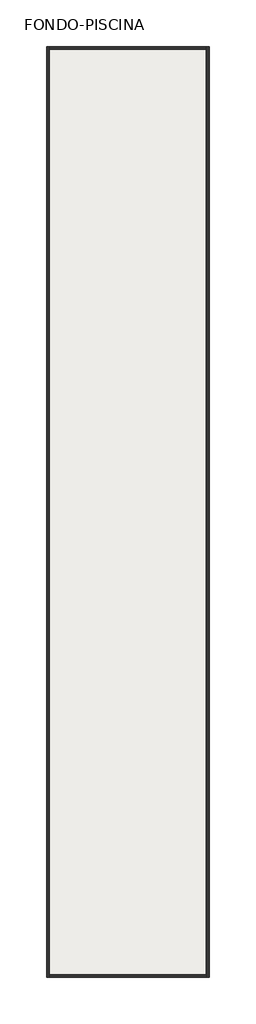
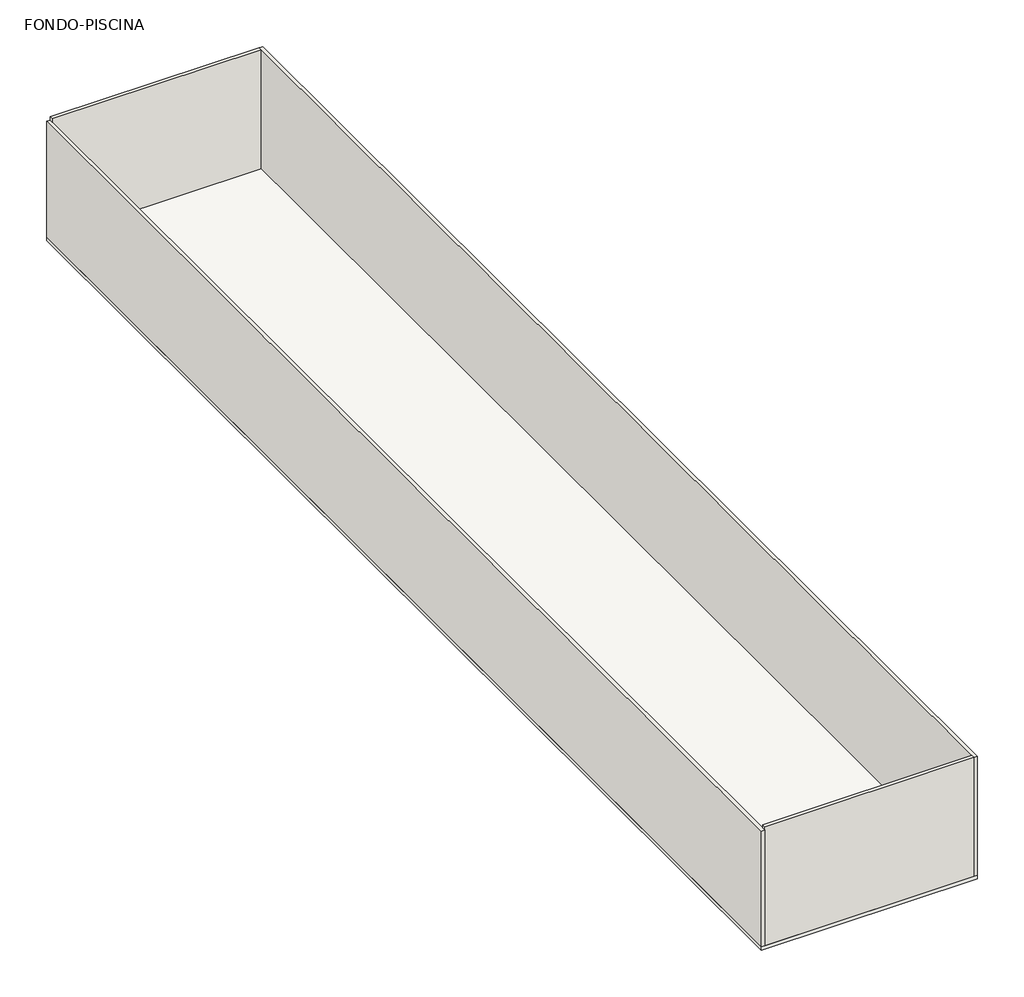
# One storey: 4 walls, 1 slab.
"""IFC4 building model written with IfcOpenShell, lengths in millimetres."""

from ifc_helpers import new_model, si_unit, origin, place, context, project, spatial, faceted_brep, element, save

model = new_model("IFC4")

# Units and contexts
model_context = context("Model", 3, world=origin())
ifc_project = project(units=[si_unit("LENGTHUNIT", "METRE", prefix="MILLI")], contexts=[model_context])

# Site, building, storey
site = spatial("IfcSite", under=ifc_project)
building = spatial("IfcBuilding", under=site)
storey = spatial("IfcBuildingStorey", under=building, Name="FONDO-PISCINA", Elevation=-1800.0)

# Slab
placement = place(None, origin())
element("IfcSlab", 1, ObjectType="ACABADO SUELO VASO PISC_PABLO", at=placement, inside=storey, context=model_context, shape_type="Brep", body=[
    faceted_brep([(-32840.0, -152.5, -1850.0), (-29750.0, -152.5, -1850.0), (-29750.0, -17847.5, -1850.0), (-32840.0, -17847.5, -1850.0), (-32840.0, -152.5, -1800.0), (-32840.0, -17847.5, -1800.0), (-32790.0, -17847.5, -1800.0), (-29800.0, -17847.5, -1800.0), (-29750.0, -17847.5, -1800.0), (-29750.0, -152.5, -1800.0), (-29800.0, -152.5, -1800.0), (-32790.0, -152.5, -1800.0)], [[[0, 1, 2, 3]], [[4, 5, 6, 7, 8, 9, 10, 11]], [[1, 0, 4, 11, 10, 9]], [[3, 2, 8, 7, 6, 5]], [[2, 1, 9, 8]], [[0, 3, 5, 4]]]),
])

# Walls
element("IfcWall", 2, ObjectType="ACABADO MURO VASO PISCINA_PABLO", at=placement, inside=storey, context=model_context, shape_type="Brep", body=[
    faceted_brep([(-29750.0, -17847.5, -1800.0), (-29750.0, -152.5, -1800.0), (-29750.0, -152.5, 0.0), (-29750.0, -17847.5, 0.0), (-29800.0, -17847.5, -1800.0), (-29800.0, -17847.5, 0.0), (-29800.0, -17797.5, 0.0), (-29800.0, -202.5, 0.0), (-29800.0, -152.5, 0.0), (-29800.0, -152.5, -1800.0), (-29800.0, -202.5, -1800.0), (-29800.0, -17797.5, -1800.0)], [[[0, 1, 2, 3]], [[4, 5, 6, 7, 8, 9, 10, 11]], [[1, 0, 4, 11, 10, 9]], [[2, 1, 9, 8]], [[3, 2, 8, 7, 6, 5]], [[0, 3, 5, 4]]]),
])
element("IfcWall", 3, ObjectType="ACABADO MURO VASO PISCINA_PABLO", at=placement, inside=storey, context=model_context, shape_type="Brep", body=[
    faceted_brep([(-29800.0, -17847.5, 0.0), (-32790.0, -17847.5, 0.0), (-32790.0, -17847.5, -50.0), (-32790.0, -17847.5, -1800.0), (-29800.0, -17847.5, -1800.0), (-32790.0, -17797.5, 0.0), (-29800.0, -17797.5, 0.0), (-29800.0, -17797.5, -1800.0), (-32790.0, -17797.5, -1800.0)], [[[0, 1, 2, 3, 4]], [[5, 6, 7, 8]], [[1, 0, 6, 5]], [[4, 3, 8, 7]], [[6, 0, 4, 7]], [[1, 5, 8, 3, 2]]]),
])
element("IfcWall", 4, ObjectType="ACABADO MURO VASO PISCINA_PABLO", at=placement, inside=storey, context=model_context, shape_type="Brep", body=[
    faceted_brep([(-29800.0, -202.5, 0.0), (-32790.0, -202.5, 0.0), (-32790.0, -202.5, -1800.0), (-29800.0, -202.5, -1800.0), (-32790.0, -152.5, 0.0), (-29800.0, -152.5, 0.0), (-29800.0, -152.5, -1800.0), (-32790.0, -152.5, -1800.0), (-32790.0, -152.5, -50.0)], [[[0, 1, 2, 3]], [[4, 5, 6, 7, 8]], [[1, 0, 5, 4]], [[3, 2, 7, 6]], [[5, 0, 3, 6]], [[1, 4, 8, 7, 2]]]),
])
element("IfcWall", 5, ObjectType="ACABADO MURO VASO PISCINA_PABLO", at=placement, inside=storey, context=model_context, shape_type="Brep", body=[
    faceted_brep([(-32790.0, -17847.5, -1800.0), (-32790.0, -17797.5, -1800.0), (-32790.0, -202.5, -1800.0), (-32790.0, -152.5, -1800.0), (-32790.0, -152.5, -50.0), (-32790.0, -17847.5, -50.0), (-32840.0, -17847.5, -1800.0), (-32840.0, -17847.5, -50.0), (-32840.0, -152.5, -50.0), (-32840.0, -152.5, -1800.0)], [[[0, 1, 2, 3, 4, 5]], [[6, 7, 8, 9]], [[3, 2, 1, 0, 6, 9]], [[4, 3, 9, 8]], [[5, 4, 8, 7]], [[0, 5, 7, 6]]]),
])

save(model, "model.ifc")

# Revit data of these elements
# Project information
#   Fecha de emisión de proyecto = "Fecha de emisión"
#   Estado de proyecto = "Estado de proyecto"
#   Nombre de cliente = "Propietario"
#   Dirección de proyecto = "Introduzca dirección aquí"
#   Nombre de proyecto = "Nombre de proyecto"
#   Número de proyecto = "0001"
# Grids (mm)
#   "10": line (-29500, 9189.325) -> (-29500, -29213.653)
#   "1": line (-33000, 9189.325) -> (-33000, -29213.653)
#   "B": line (7688.401, -13500) -> (-37134.551, -13500)
#   "A": line (7688.401, -18000) -> (-37134.551, -18000)
#   "BC": line (7688.401, -9000) -> (-37134.551, -9000)
#   "C": line (7688.401, -4500) -> (-37134.551, -4500)
#   "D": line (7688.401, 0) -> (-37134.551, 0)
#   "6": line (0, 9189.325) -> (0, -29213.653)
#   "56": line (-6000, 9189.325) -> (-6000, -29213.653)
#   "5": line (-9000, 9189.325) -> (-9000, -29213.653)
#   "4": line (-12000, 9189.325) -> (-12000, -29213.653)
#   "3": line (-21000, 9189.325) -> (-21000, -29213.653)
#   "2": line (-24000, 9189.325) -> (-24000, -29213.653)
#   "12": line (-27000, 9189.325) -> (-27000, -29213.653)
# Type "ACABADO SUELO VASO PISC_PABLO"
#   Keynote = "S.4.2"
#   Function = 0
#   Layers, outside or top first: 0.03 m "Piedra caliza acabado" (function 5); 0.02 m "Mortero agarre" (function 4)
# Type "ACABADO MURO VASO PISCINA_PABLO"
#   Keynote = "Me.1.1"
#   Layers, outside or top first: 0.03 m "Piedra caliza acabado" (function 5); 0.02 m "Mortero agarre" (function 4); 0.00 m "Membrana impermeabilizante" (function 100)
# Element 1 (IfcSlab, "ACABADO SUELO VASO PISC_PABLO")
#   Comments = ""
#   built-in parameter 1001955 = 3.14159 (stored number, unit not read)
#   Height Offset From Level = 0.00 m
#   built-in parameter 1001954 = 1
#   Phase Created = Nueva construcción
#   Materials on its faces: "Mortero agarre", "Piedra caliza acabado"
# Element 2 (IfcWall, "ACABADO MURO VASO PISCINA_PABLO")
#   Top Offset = 0.00 m
#   Base Offset = 0.00 m
#   wall height = 1.80 m
#   Phase Created = Nueva construcción
#   Base Constraint = FONDO-PISCINA
#   Top Constraint = ACCESO
#   Materials on its faces: "Piedra caliza acabado", "Mortero agarre"
# Elements 3, 4 (IfcWall, "ACABADO MURO VASO PISCINA_PABLO")
#   built-in parameter 1001111 = -0.05 m
#   Top Offset = 0.00 m
#   Base Offset = -0.05 m
#   wall height = 1.85 m
#   Phase Created = Nueva construcción
#   Base Constraint = FONDO-PISCINA
#   Top Constraint = ACCESO
#   Materials on its faces: "Piedra caliza acabado", "Mortero agarre"
# Element 5 (IfcWall, "ACABADO MURO VASO PISCINA_PABLO")
#   Top Offset = -0.05 m
#   Base Offset = 0.00 m
#   wall height = 1.75 m
#   Phase Created = Nueva construcción
#   Base Constraint = FONDO-PISCINA
#   Top Constraint = ACCESO
#   Materials on its faces: "Piedra caliza acabado", "Mortero agarre"
# Materials
#   "Piedra caliza acabado": class "Piedra", colour RGB 120 120 120, transparency 0, Keynote = "3", Comments = "Revestimiento interior (2 cm)", Description = "Caliza, áspero, sillar tosco", Cost = 0
#   "Mortero agarre": class "Varios", colour RGB 127 127 127, transparency 0, Comments = "(1,5 cm)", Description = "mortero hidrófugo", Cost = 0
#   "Membrana impermeabilizante": class "Plástico", colour RGB 127 127 127, transparency 0, Comments = "Lámina (1,2 mm) armada con fibra de vidrio", Description = "Acabado exterior, cubierta", Cost = 0
